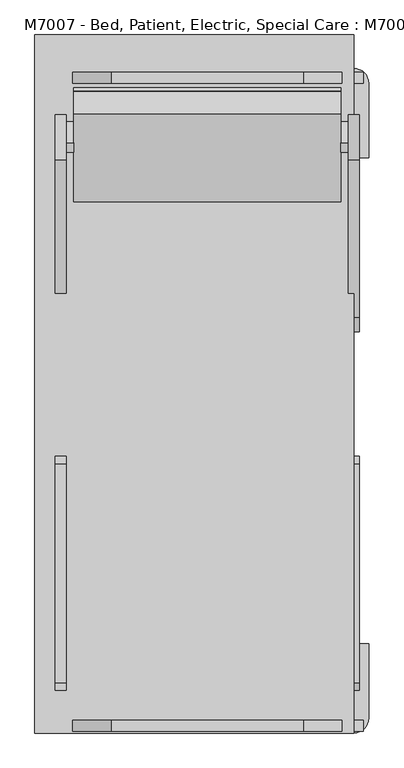
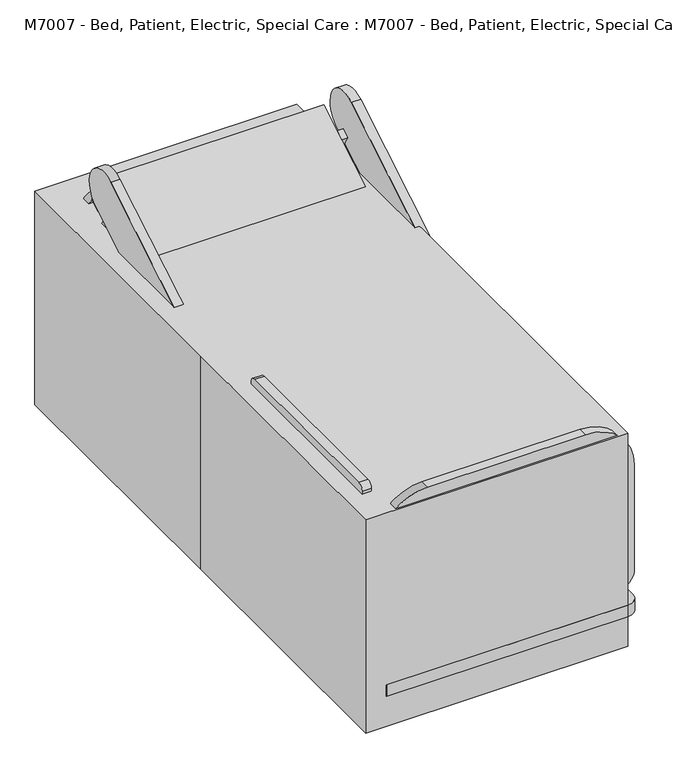
"""IFC4 building model written with IfcOpenShell, lengths in millimetres: proxy geometry, M7007 - Bed, Patient, Electric, Special Care : M7007 - Bed, Patient, Electric, Special Care."""

from ifc_helpers import new_model, si_unit, point, frame, frame_2d, origin, origin_with_axes, place, context, project, spatial, polyline, circle_curve, trimmed, segment, composite_curve, outline, extrude, source, transform, mapped, element, save


def m7007_bed_patient_electric_special_care_m7007_bed_patient_e65fd407(model_context):
    return source(origin(), model_context, "Body", "SweptSolid", [
        extrude(outline(polyline([(0.0, -38.1), (0.0, 0.0), (25.4, 0.0), (25.4, -38.1), (0.0, -38.1)])), frame((501.65, 512.7423906, 664.2653407), z_axis=(0.0, -0.499999999999999, 0.8660254037844393), x_axis=(1.0, 0.0, 0.0)), (0.0, 0.0, 1.0), 177.8),
        extrude(outline(composite_curve([segment(polyline([(871.8063934, 1040.3170455), (332.9481698, 716.5383597)]), True, "CONTINUOUS"), segment(trimmed(circle_curve(frame_2d((280.6203014, 803.6265574)), 101.6), [point((332.9481698, 716.5383597))], [point((228.292433, 890.7147552))], False, "CARTESIAN"), True, "CONTINUOUS"), segment(polyline([(228.292433, 890.7147552), (767.1506566, 1214.493441)]), True, "CONTINUOUS"), segment(trimmed(circle_curve(frame_2d((819.478525, 1127.4052432)), 101.6), [point((767.1506566, 1214.493441))], [point((871.8063934, 1040.3170455))], False, "CARTESIAN"), True, "CONTINUOUS")], self_intersect=False)), frame((527.05, 0.0, 0.0), z_axis=(1.0, 0.0, 0.0), x_axis=(0.0, 1.0, 0.0)), (0.0, 0.0, 1.0), 38.1),
        extrude(outline(polyline([(0.0, -38.1), (0.0, 0.0), (25.4, 0.0), (25.4, -38.1), (0.0, -38.1)])), frame((501.65, 914.5832957, 908.7403407), z_axis=(0.0, -0.49999999999999634, 0.8660254037844408), x_axis=(1.0, 0.0, 0.0)), (0.0, 0.0, 1.0), 177.8),
        extrude(outline(composite_curve([segment(polyline([(871.8063934, 1040.3170455), (332.9481698, 716.5383597)]), True, "CONTINUOUS"), segment(trimmed(circle_curve(frame_2d((280.6203014, 803.6265574)), 101.6), [point((332.9481698, 716.5383597))], [point((228.292433, 890.7147552))], False, "CARTESIAN"), True, "CONTINUOUS"), segment(polyline([(228.292433, 890.7147552), (767.1506566, 1214.493441)]), True, "CONTINUOUS"), segment(trimmed(circle_curve(frame_2d((819.478525, 1127.4052432)), 101.6), [point((767.1506566, 1214.493441))], [point((871.8063934, 1040.3170455))], False, "CARTESIAN"), True, "CONTINUOUS")], self_intersect=False)), frame((-476.25, 0.0, 0.0), z_axis=(1.0, 0.0, 0.0), x_axis=(0.0, 1.0, 0.0)), (0.0, 0.0, 1.0), 38.1),
        extrude(outline(polyline([(0.0, -38.1), (0.0, 0.0), (25.4, 0.0), (25.4, -38.1), (0.0, -38.1)])), frame((-412.75, 479.7468227, 645.2153407), z_axis=(0.0, -0.499999999999999, 0.8660254037844393), x_axis=(-1.0, 0.0, 0.0)), (0.0, 0.0, 1.0), 177.8),
        extrude(outline(polyline([(0.0, -38.1), (0.0, 0.0), (25.4, 0.0), (25.4, -38.1), (0.0, -38.1)])), frame((-412.75, 881.5877278, 889.6903407), z_axis=(0.0, -0.49999999999999634, 0.8660254037844408), x_axis=(-1.0, 0.0, 0.0)), (0.0, 0.0, 1.0), 177.8),
        extrude(outline(composite_curve([segment(polyline([(-857.3563812, 519.7510043), (-857.3563812, 634.0510043), (-1022.4563812, 634.0510043)]), True, "CONTINUOUS"), segment(trimmed(circle_curve(frame_2d((-1022.4563812, 659.4510043)), 25.4), [point((-1022.4563812, 634.0510043))], [point((-1047.8563812, 659.4510043))], False, "CARTESIAN"), True, "CONTINUOUS"), segment(polyline([(-1047.8563812, 659.4510043), (-1047.8563812, 748.3510043)]), True, "CONTINUOUS"), segment(trimmed(circle_curve(frame_2d((-1022.4563812, 748.3510043)), 25.4), [point((-1047.8563812, 748.3510043))], [point((-1022.4563812, 773.7510043))], False, "CARTESIAN"), True, "CONTINUOUS"), segment(polyline([(-1022.4563812, 773.7510043), (-273.1563812, 773.7510043)]), True, "CONTINUOUS"), segment(trimmed(circle_curve(frame_2d((-273.1563812, 748.3510043)), 25.4), [point((-273.1563812, 773.7510043))], [point((-247.7563812, 748.3510043))], False, "CARTESIAN"), True, "CONTINUOUS"), segment(polyline([(-247.7563812, 748.3510043), (-247.7563812, 519.7510043), (-857.3563812, 519.7510043)]), True, "CONTINUOUS")], self_intersect=False)), frame((527.05, 0.0, 0.0), z_axis=(1.0, 0.0, 0.0), x_axis=(0.0, 1.0, 0.0)), (0.0, 0.0, 1.0), 38.1),
        extrude(outline(polyline([(501.65, -837.1721819), (501.65, -799.0721819), (527.05, -799.0721819), (527.05, -837.1721819), (501.65, -837.1721819)])), frame((0.0, 0.0, 595.9510043), z_axis=(0.0, 0.0, 1.0), x_axis=(1.0, 0.0, 0.0)), (0.0, 0.0, 1.0), 177.8),
        extrude(outline(polyline([(501.65, -329.1721819), (501.65, -291.0721819), (527.05, -291.0721819), (527.05, -329.1721819), (501.65, -329.1721819)])), frame((0.0, 0.0, 595.9510043), z_axis=(0.0, 0.0, 1.0), x_axis=(1.0, 0.0, 0.0)), (0.0, 0.0, 1.0), 177.8),
        extrude(outline(composite_curve([segment(polyline([(-857.3563812, 723.110535), (-857.3563812, 837.410535), (-1022.4563812, 837.410535)]), True, "CONTINUOUS"), segment(trimmed(circle_curve(frame_2d((-1022.4563812, 862.810535)), 25.4), [point((-1022.4563812, 837.410535))], [point((-1047.8563812, 862.810535))], False, "CARTESIAN"), True, "CONTINUOUS"), segment(polyline([(-1047.8563812, 862.810535), (-1047.8563812, 951.710535)]), True, "CONTINUOUS"), segment(trimmed(circle_curve(frame_2d((-1022.4563812, 951.710535)), 25.4), [point((-1047.8563812, 951.710535))], [point((-1022.4563812, 977.110535))], False, "CARTESIAN"), True, "CONTINUOUS"), segment(polyline([(-1022.4563812, 977.110535), (-273.1563812, 977.110535)]), True, "CONTINUOUS"), segment(trimmed(circle_curve(frame_2d((-273.1563812, 951.710535)), 25.4), [point((-273.1563812, 977.110535))], [point((-247.7563812, 951.710535))], False, "CARTESIAN"), True, "CONTINUOUS"), segment(polyline([(-247.7563812, 951.710535), (-247.7563812, 723.110535), (-857.3563812, 723.110535)]), True, "CONTINUOUS")], self_intersect=False)), frame((-476.25, 0.0, 0.0), z_axis=(1.0, 0.0, 0.0), x_axis=(0.0, 1.0, 0.0)), (0.0, 0.0, 1.0), 38.1),
        extrude(outline(polyline([(-412.75, -799.0721819), (-412.75, -837.1721819), (-438.15, -837.1721819), (-438.15, -799.0721819), (-412.75, -799.0721819)])), frame((0.0, 0.0, 595.9510043), z_axis=(0.0, 0.0, 1.0), x_axis=(1.0, 0.0, 0.0)), (0.0, 0.0, 1.0), 177.8),
        extrude(outline(polyline([(-412.75, -291.0721819), (-412.75, -329.1721819), (-438.15, -329.1721819), (-438.15, -291.0721819), (-412.75, -291.0721819)])), frame((0.0, 0.0, 595.9510043), z_axis=(0.0, 0.0, 1.0), x_axis=(1.0, 0.0, 0.0)), (0.0, 0.0, 1.0), 177.8),
        extrude(outline(polyline([(977.9, 383.6291673), (825.4956539, 383.6291673), (825.4956539, 850.8553975), (977.9, 942.4291673), (977.9, 383.6291673)])), frame((-107.95, 0.0, 0.0), z_axis=(1.0, 0.0, 0.0), x_axis=(0.0, 1.0, 0.0)), (0.0, 0.0, 1.0), 304.8),
        extrude(outline(polyline([(-23.330399, 621.3510043), (-1140.930399, 621.3510043), (-1140.930399, 773.7510043), (5.8953565, 773.7510043), (152.3074458, 715.4521116), (289.44733, 739.6335733), (922.2017014, 1119.8307566), (1000.693504, 989.19846), (343.7278675, 594.4536809), (136.1437733, 557.8510043), (-23.330399, 621.3510043)])), frame((-412.75, 0.0, 0.0), z_axis=(1.0, 0.0, 0.0), x_axis=(0.0, 1.0, 0.0)), (0.0, 0.0, 1.0), 914.4),
        extrude(outline(composite_curve([segment(polyline([(988.8271945, 374.65), (988.8271945, -285.75)]), True, "CONTINUOUS"), segment(trimmed(circle_curve(frame_2d((785.6271945, -285.75)), 203.2), [point((988.8271945, -285.75))], [point((785.6271945, -488.95))], False, "CARTESIAN"), True, "CONTINUOUS"), segment(polyline([(785.6271945, -488.95), (329.8584688, -488.95)]), True, "CONTINUOUS"), segment(trimmed(circle_curve(frame_2d((329.8584688, -412.75)), 76.2), [point((329.8584688, -488.95))], [point((253.6584688, -412.75))], False, "CARTESIAN"), True, "CONTINUOUS"), segment(polyline([(253.6584688, -412.75), (253.6584688, 501.65)]), True, "CONTINUOUS"), segment(trimmed(circle_curve(frame_2d((329.8584688, 501.65)), 76.2), [point((253.6584688, 501.65))], [point((329.8584688, 577.85))], False, "CARTESIAN"), True, "CONTINUOUS"), segment(polyline([(329.8584688, 577.85), (785.6271945, 577.85)]), True, "CONTINUOUS"), segment(trimmed(circle_curve(frame_2d((785.6271945, 374.65)), 203.2), [point((785.6271945, 577.85))], [point((988.8271945, 374.65))], False, "CARTESIAN"), True, "CONTINUOUS")], self_intersect=False)), frame((0.0, 1028.7, 0.0), z_axis=(0.0, 1.0, 0.0), x_axis=(0.0, 0.0, 1.0)), (0.0, 0.0, 1.0), 38.1),
        extrude(outline(polyline([(260.35, -330.2), (-171.45, -330.2), (-171.45, -76.2), (260.35, -76.2), (260.35, -330.2)])), frame((0.0, 0.0, 180.975), z_axis=(0.0, 0.0, 1.0), x_axis=(1.0, 0.0, 0.0)), (0.0, 0.0, 1.0), 414.9760043),
        extrude(outline(polyline([(-1140.930399, 595.9510043), (-1140.930399, 621.3510043), (-67.3244895, 621.3510043), (42.6607368, 557.8510043), (282.8107839, 557.8510043), (1000.693504, 989.19846), (1013.7754711, 967.4264105), (289.8548273, 532.4510043), (35.8548273, 532.4510043), (-74.130399, 595.9510043), (-1140.930399, 595.9510043)])), frame((-412.75, 0.0, 0.0), z_axis=(1.0, 0.0, 0.0), x_axis=(0.0, 1.0, 0.0)), (0.0, 0.0, 1.0), 914.4),
        extrude(outline(composite_curve([segment(trimmed(circle_curve(frame_2d((952.3599321, 51.5042315)), 51.5042315), [point((900.8557006, 51.5042315))], [point((1003.8641636, 51.5042315))], False, "CARTESIAN"), True, "CONTINUOUS"), segment(trimmed(circle_curve(frame_2d((952.3599321, 51.5042315)), 51.5042315), [point((1003.8641636, 51.5042315))], [point((900.8557006, 51.5042315))], False, "CARTESIAN"), True, "CONTINUOUS")], self_intersect=False)), frame((-438.15, 0.0, 0.0), z_axis=(1.0, 0.0, 0.0), x_axis=(0.0, 1.0, 0.0)), (0.0, 0.0, 1.0), 25.4),
        extrude(outline(composite_curve([segment(trimmed(circle_curve(frame_2d((952.3599321, 51.5042315)), 51.5042315), [point((900.8557006, 51.5042315))], [point((1003.8641636, 51.5042315))], False, "CARTESIAN"), True, "CONTINUOUS"), segment(trimmed(circle_curve(frame_2d((952.3599321, 51.5042315)), 51.5042315), [point((1003.8641636, 51.5042315))], [point((900.8557006, 51.5042315))], False, "CARTESIAN"), True, "CONTINUOUS")], self_intersect=False)), frame((488.95, 0.0, 0.0), z_axis=(1.0, 0.0, 0.0), x_axis=(0.0, 1.0, 0.0)), (0.0, 0.0, 1.0), 25.4),
        extrude(outline(composite_curve([segment(trimmed(circle_curve(frame_2d((-1066.6599321, 51.5042315)), 51.5042315), [point((-1015.1557006, 51.5042315))], [point((-1118.1641636, 51.5042315))], False, "CARTESIAN"), True, "CONTINUOUS"), segment(trimmed(circle_curve(frame_2d((-1066.6599321, 51.5042315)), 51.5042315), [point((-1118.1641636, 51.5042315))], [point((-1015.1557006, 51.5042315))], False, "CARTESIAN"), True, "CONTINUOUS")], self_intersect=False)), frame((488.95, 0.0, 0.0), z_axis=(1.0, 0.0, 0.0), x_axis=(0.0, 1.0, 0.0)), (0.0, 0.0, 1.0), 25.4),
        extrude(outline(composite_curve([segment(polyline([(964.9863453, 60.4258647), (959.99125, 48.3666377)]), True, "CONTINUOUS"), segment(trimmed(circle_curve(frame_2d((950.7378796, 50.8460708)), 9.5797939), [point((959.99125, 48.3666377))], [point((941.1580857, 50.8460708))], False, "CARTESIAN"), True, "CONTINUOUS"), segment(polyline([(941.1580857, 50.8460708), (941.1580857, 108.9715457), (950.8356274, 130.175), (981.1868486, 130.175)]), True, "CONTINUOUS"), segment(trimmed(circle_curve(frame_2d((981.1868486, 121.6954559)), 8.4795441), [point((981.1868486, 130.175))], [point((989.0209258, 118.4504749))], False, "CARTESIAN"), True, "CONTINUOUS"), segment(polyline([(989.0209258, 118.4504749), (964.9863453, 60.4258647)]), True, "CONTINUOUS")], self_intersect=False)), frame((482.6, 0.0, 0.0), z_axis=(1.0, 0.0, 0.0), x_axis=(0.0, 1.0, 0.0)), (0.0, 0.0, 1.0), 38.1),
        extrude(outline(composite_curve([segment(trimmed(circle_curve(frame_2d((952.3599321, 51.5042315)), 51.5042315), [point((900.8557006, 51.5042315))], [point((1003.8641636, 51.5042315))], False, "CARTESIAN"), True, "CONTINUOUS"), segment(trimmed(circle_curve(frame_2d((952.3599321, 51.5042315)), 51.5042315), [point((1003.8641636, 51.5042315))], [point((900.8557006, 51.5042315))], False, "CARTESIAN"), True, "CONTINUOUS")], self_intersect=False)), frame((488.95, 0.0, 0.0), z_axis=(1.0, 0.0, 0.0), x_axis=(0.0, 1.0, 0.0)), (0.0, 0.0, 1.0), 25.4),
        extrude(outline(composite_curve([segment(polyline([(964.9863453, 60.4258647), (959.99125, 48.3666377)]), True, "CONTINUOUS"), segment(trimmed(circle_curve(frame_2d((950.7378796, 50.8460708)), 9.5797939), [point((959.99125, 48.3666377))], [point((941.1580857, 50.8460708))], False, "CARTESIAN"), True, "CONTINUOUS"), segment(polyline([(941.1580857, 50.8460708), (941.1580857, 108.9715457), (950.8356274, 130.175), (981.1868486, 130.175)]), True, "CONTINUOUS"), segment(trimmed(circle_curve(frame_2d((981.1868486, 121.6954559)), 8.4795441), [point((981.1868486, 130.175))], [point((989.0209258, 118.4504749))], False, "CARTESIAN"), True, "CONTINUOUS"), segment(polyline([(989.0209258, 118.4504749), (964.9863453, 60.4258647)]), True, "CONTINUOUS")], self_intersect=False)), frame((-444.5, 0.0, 0.0), z_axis=(1.0, 0.0, 0.0), x_axis=(0.0, 1.0, 0.0)), (0.0, 0.0, 1.0), 38.1),
        extrude(outline(composite_curve([segment(trimmed(circle_curve(frame_2d((952.3599321, 51.5042315)), 51.5042315), [point((900.8557006, 51.5042315))], [point((1003.8641636, 51.5042315))], False, "CARTESIAN"), True, "CONTINUOUS"), segment(trimmed(circle_curve(frame_2d((952.3599321, 51.5042315)), 51.5042315), [point((1003.8641636, 51.5042315))], [point((900.8557006, 51.5042315))], False, "CARTESIAN"), True, "CONTINUOUS")], self_intersect=False)), frame((-438.15, 0.0, 0.0), z_axis=(1.0, 0.0, 0.0), x_axis=(0.0, 1.0, 0.0)), (0.0, 0.0, 1.0), 25.4),
        extrude(outline(composite_curve([segment(polyline([(-1079.2863453, 60.4258647), (-1103.3209258, 118.4504749)]), True, "CONTINUOUS"), segment(trimmed(circle_curve(frame_2d((-1095.4868486, 121.6954559)), 8.4795441), [point((-1103.3209258, 118.4504749))], [point((-1095.4868486, 130.175))], False, "CARTESIAN"), True, "CONTINUOUS"), segment(polyline([(-1095.4868486, 130.175), (-1065.1356274, 130.175), (-1055.4580857, 108.9715457), (-1055.4580857, 50.8460708)]), True, "CONTINUOUS"), segment(trimmed(circle_curve(frame_2d((-1065.0378796, 50.8460708)), 9.5797939), [point((-1055.4580857, 50.8460708))], [point((-1074.29125, 48.3666377))], False, "CARTESIAN"), True, "CONTINUOUS"), segment(polyline([(-1074.29125, 48.3666377), (-1079.2863453, 60.4258647)]), True, "CONTINUOUS")], self_intersect=False)), frame((482.6, 0.0, 0.0), z_axis=(1.0, 0.0, 0.0), x_axis=(0.0, 1.0, 0.0)), (0.0, 0.0, 1.0), 38.1),
        extrude(outline(composite_curve([segment(trimmed(circle_curve(frame_2d((-1066.6599321, 51.5042315)), 51.5042315), [point((-1015.1557006, 51.5042315))], [point((-1118.1641636, 51.5042315))], False, "CARTESIAN"), True, "CONTINUOUS"), segment(trimmed(circle_curve(frame_2d((-1066.6599321, 51.5042315)), 51.5042315), [point((-1118.1641636, 51.5042315))], [point((-1015.1557006, 51.5042315))], False, "CARTESIAN"), True, "CONTINUOUS")], self_intersect=False)), frame((488.95, 0.0, 0.0), z_axis=(1.0, 0.0, 0.0), x_axis=(0.0, 1.0, 0.0)), (0.0, 0.0, 1.0), 25.4),
        extrude(outline(composite_curve([segment(polyline([(-1079.2863453, 60.4258647), (-1103.3209258, 118.4504749)]), True, "CONTINUOUS"), segment(trimmed(circle_curve(frame_2d((-1095.4868486, 121.6954559)), 8.4795441), [point((-1103.3209258, 118.4504749))], [point((-1095.4868486, 130.175))], False, "CARTESIAN"), True, "CONTINUOUS"), segment(polyline([(-1095.4868486, 130.175), (-1065.1356274, 130.175), (-1055.4580857, 108.9715457), (-1055.4580857, 50.8460708)]), True, "CONTINUOUS"), segment(trimmed(circle_curve(frame_2d((-1065.0378796, 50.8460708)), 9.5797939), [point((-1055.4580857, 50.8460708))], [point((-1074.29125, 48.3666377))], False, "CARTESIAN"), True, "CONTINUOUS"), segment(polyline([(-1074.29125, 48.3666377), (-1079.2863453, 60.4258647)]), True, "CONTINUOUS")], self_intersect=False)), frame((-444.5, 0.0, 0.0), z_axis=(1.0, 0.0, 0.0), x_axis=(0.0, 1.0, 0.0)), (0.0, 0.0, 1.0), 38.1),
        extrude(outline(composite_curve([segment(trimmed(circle_curve(frame_2d((-1066.6599321, 51.5042315)), 51.5042315), [point((-1015.1557006, 51.5042315))], [point((-1118.1641636, 51.5042315))], False, "CARTESIAN"), True, "CONTINUOUS"), segment(trimmed(circle_curve(frame_2d((-1066.6599321, 51.5042315)), 51.5042315), [point((-1118.1641636, 51.5042315))], [point((-1015.1557006, 51.5042315))], False, "CARTESIAN"), True, "CONTINUOUS")], self_intersect=False)), frame((-438.15, 0.0, 0.0), z_axis=(1.0, 0.0, 0.0), x_axis=(0.0, 1.0, 0.0)), (0.0, 0.0, 1.0), 25.4),
        extrude(outline(polyline([(260.35, 774.7), (-171.45, 774.7), (-171.45, 1028.7), (260.35, 1028.7), (260.35, 774.7)])), frame((0.0, 0.0, 180.975), z_axis=(0.0, 0.0, 1.0), x_axis=(1.0, 0.0, 0.0)), (0.0, 0.0, 1.0), 202.6541673),
        extrude(outline(polyline([(260.35, -1143.0), (-171.45, -1143.0), (-171.45, -889.0), (260.35, -889.0), (260.35, -1143.0)])), frame((0.0, 0.0, 180.975), z_axis=(0.0, 0.0, 1.0), x_axis=(1.0, 0.0, 0.0)), (0.0, 0.0, 1.0), 414.9760043),
        extrude(outline(composite_curve([segment(polyline([(988.8271945, 374.65), (988.8271945, -285.75)]), True, "CONTINUOUS"), segment(trimmed(circle_curve(frame_2d((785.6271945, -285.75)), 203.2), [point((988.8271945, -285.75))], [point((785.6271945, -488.95))], False, "CARTESIAN"), True, "CONTINUOUS"), segment(polyline([(785.6271945, -488.95), (326.7009977, -488.95)]), True, "CONTINUOUS"), segment(trimmed(circle_curve(frame_2d((326.7009977, -412.75)), 76.2), [point((326.7009977, -488.95))], [point((250.5009977, -412.75))], False, "CARTESIAN"), True, "CONTINUOUS"), segment(polyline([(250.5009977, -412.75), (250.5009977, 501.65)]), True, "CONTINUOUS"), segment(trimmed(circle_curve(frame_2d((326.7009977, 501.65)), 76.2), [point((250.5009977, 501.65))], [point((326.7009977, 577.85))], False, "CARTESIAN"), True, "CONTINUOUS"), segment(polyline([(326.7009977, 577.85), (785.6271945, 577.85)]), True, "CONTINUOUS"), segment(trimmed(circle_curve(frame_2d((785.6271945, 374.65)), 203.2), [point((785.6271945, 577.85))], [point((988.8271945, 374.65))], False, "CARTESIAN"), True, "CONTINUOUS")], self_intersect=False)), frame((0.0, -1187.45, 0.0), z_axis=(0.0, 1.0, 0.0), x_axis=(0.0, 0.0, 1.0)), (0.0, 0.0, 1.0), 38.1),
        extrude(outline(composite_curve([segment(trimmed(circle_curve(frame_2d((546.1, 1028.7)), 50.8), [point((546.1, 1079.5))], [point((596.9, 1028.7))], False, "CARTESIAN"), True, "CONTINUOUS"), segment(polyline([(596.9, 1028.7), (596.9, 774.7), (444.5, 774.7), (444.5, -889.0), (596.9, -889.0), (596.9, -1143.0)]), True, "CONTINUOUS"), segment(trimmed(circle_curve(frame_2d((546.1, -1143.0)), 50.8), [point((596.9, -1143.0))], [point((546.1, -1193.8))], False, "CARTESIAN"), True, "CONTINUOUS"), segment(polyline([(546.1, -1193.8), (-457.2, -1193.8)]), True, "CONTINUOUS"), segment(trimmed(circle_curve(frame_2d((-457.2, -1143.0)), 50.8), [point((-457.2, -1193.8))], [point((-508.0, -1143.0))], False, "CARTESIAN"), True, "CONTINUOUS"), segment(polyline([(-508.0, -1143.0), (-508.0, -889.0), (-355.6, -889.0), (-355.6, 774.7), (-508.0, 774.7), (-508.0, 1028.7)]), True, "CONTINUOUS"), segment(trimmed(circle_curve(frame_2d((-457.2, 1028.7)), 50.8), [point((-508.0, 1028.7))], [point((-457.2, 1079.5))], False, "CARTESIAN"), True, "CONTINUOUS"), segment(polyline([(-457.2, 1079.5), (546.1, 1079.5)]), True, "CONTINUOUS")], self_intersect=False)), frame((0.0, 0.0, 130.175), z_axis=(0.0, 0.0, 1.0), x_axis=(1.0, 0.0, 0.0)), (0.0, 0.0, 1.0), 50.8),
        extrude(outline(polyline([(-546.1, 1193.8), (546.1, 1193.8), (546.1, -1193.8), (-546.1, -1193.8), (-546.1, 0.0), (-546.1, 1193.8)])), origin_with_axes(), (0.0, 0.0, 1.0), 939.8),
    ])


if __name__ == "__main__":
    model = new_model("IFC4")
    model_context = context("Model", 3, world=origin())
    ifc_project = project(units=[si_unit("LENGTHUNIT", "METRE", prefix="MILLI")], contexts=[model_context])
    site = spatial("IfcSite", under=ifc_project)
    building = spatial("IfcBuilding", under=site)
    placement = place(None, origin())
    m7007_bed_patient_electric_special_care_m7007_bed_patient_shape = m7007_bed_patient_electric_special_care_m7007_bed_patient_e65fd407(model_context)
    element("IfcBuildingElementProxy", 1, Name="M7007 - Bed, Patient, Electric, Special Care : M7007 - Bed, Patient, Electric, Special Care", ObjectType="M7007 - Bed, Patient, Electric, Special Care : M7007 - Bed, Patient, Electric, Special Care", at=placement, inside=building, context=model_context, shape_type="MappedRepresentation", body=[
        mapped(m7007_bed_patient_electric_special_care_m7007_bed_patient_shape, transform((0.0, 0.0, 0.0), x_axis=(1.0, 0.0, 0.0), y_axis=(0.0, 1.0, 0.0), z_axis=(0.0, 0.0, 1.0))),
    ])
    save(model, "model.ifc")

# Revit data of these elements
# Type "M7007 - Bed, Patient, Electric, Special Care : M7007 - Bed, Patient, Electric, Special Care"
#   Watts2 = "0"
#   Watts1 = "1200"
#   Unit_Issue = "EA"
#   UTIL_6_Misc = "-"
#   UTIL_5_NonMedGas = "-"
#   UTIL_4_MiscGas = "-"
#   UTIL_3_MedGas = "-"
#   UTIL_2_Elec = "A"
#   UTIL_1_WaterDrain = "-"
#   Nomenclature = "Bed, Patient, Electric, Special Care"
#   NSN = "6530"
#   Location [instance default] = ""
#   JSN = "M7007"
#   Fund_Source_VA = "-"
#   Fund_Source_Navy = "-"
#   Fund_Source_Army = "-"
#   Fund_Source_AF = "-"
#   ELEC_Volts2 = "0"
#   ELEC_Volts1 = "120"
#   ELEC_Phase2 = "0"
#   ELEC_Phase1 = "1"
#   ELEC_HertzSwitch = "0"
#   ELEC_HertzDependent = "-1"
#   ELEC_Hertz = "60"
#   ELEC_Amps2 = "0"
#   ELEC_Amps1 = "10"
#   DetailDescription = "Electric patient bed for special care areas. Unit features a control panel for the patients operation, IV rod locations and a full range of positions. Includes safety sides, thermal overload protection in the motors, provisions for chest x-rays and fluoroscopy. Bed deck is x-ray translucent."
#   CAT_VA = "C"
#   CAT_Navy = "C"
#   CAT_IHS = "-"
#   CAT_Army = "C"
#   CAT_AF = "C"
#   BTUperhour = "0"
#   Weight_IP = 600
#   DIM_Width_IP = 3' - 7"
#   DIM_Height_IP = 3' - 1"
#   DIM_Depth_IP = 7' - 10"
#   head / foor board [instance default] = none
#   frame [instance default] = none
#   caster material [instance default] = none
# Element 1 (IfcBuildingElementProxy, "M7007 - Bed, Patient, Electric, Special Care : M7007 - Bed, Patient, Electric, Special Care")
#   Materials on its faces: "EquipSpace"
# Materials
#   "EquipSpace": class "Unassigned", colour RGB 221 217 195, transparency 0.5
